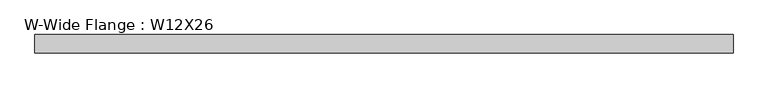
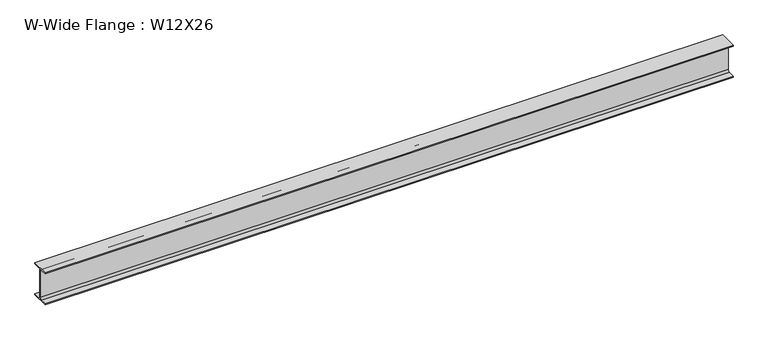
"""IFC4 building model written with IfcOpenShell, lengths in millimetres: beam geometry, W-Wide Flange : W12X26."""

from ifc_helpers import new_model, si_unit, point, frame, frame_2d, origin, place, context, project, spatial, polyline, circle_curve, trimmed, segment, composite_curve, outline, extrude, source, transform, mapped, element, save


def w_wide_flange_w12x26_2b793ae1(model_context):
    return source(origin(), model_context, "Body", "SweptSolid", [
        extrude(outline(composite_curve([segment(polyline([(82.4011719, -145.5539063), (82.4011719, -155.178125), (-82.4011719, -155.178125), (-82.4011719, -145.5539063), (-20.2902344, -145.5539063)]), True, "CONTINUOUS"), segment(trimmed(circle_curve(frame_2d((-20.2902344, -128.190625)), 17.3632812), [point((-20.2902344, -145.5539063))], [point((-2.9269531, -128.190625))], True, "CARTESIAN"), True, "CONTINUOUS"), segment(polyline([(-2.9269531, -128.190625), (-2.9269531, 128.190625)]), True, "CONTINUOUS"), segment(trimmed(circle_curve(frame_2d((-20.2902344, 128.190625)), 17.3632812), [point((-2.9269531, 128.190625))], [point((-20.2902344, 145.5539062))], True, "CARTESIAN"), True, "CONTINUOUS"), segment(polyline([(-20.2902344, 145.5539062), (-82.4011719, 145.5539062), (-82.4011719, 155.178125), (82.4011719, 155.178125), (82.4011719, 145.5539062), (20.2902344, 145.5539062)]), True, "CONTINUOUS"), segment(trimmed(circle_curve(frame_2d((20.2902344, 128.190625)), 17.3632812), [point((20.2902344, 145.5539062))], [point((2.9269531, 128.190625))], True, "CARTESIAN"), True, "CONTINUOUS"), segment(polyline([(2.9269531, 128.190625), (2.9269531, -128.190625)]), True, "CONTINUOUS"), segment(trimmed(circle_curve(frame_2d((20.2902344, -128.190625)), 17.3632812), [point((2.9269531, -128.190625))], [point((20.2902344, -145.5539063))], True, "CARTESIAN"), True, "CONTINUOUS"), segment(polyline([(20.2902344, -145.5539063), (82.4011719, -145.5539063)]), True, "CONTINUOUS")], self_intersect=False)), frame((-3159.4630915, 0.0, 0.0), z_axis=(1.0, 0.0, 0.0), x_axis=(0.0, 1.0, 0.0)), (0.0, 0.0, 1.0), 6318.926183),
    ])


if __name__ == "__main__":
    model = new_model("IFC4")
    model_context = context("Model", 3, world=origin())
    ifc_project = project(units=[si_unit("LENGTHUNIT", "METRE", prefix="MILLI")], contexts=[model_context])
    site = spatial("IfcSite", under=ifc_project)
    building = spatial("IfcBuilding", under=site)
    placement = place(None, origin())
    w_wide_flange_w12x26_shape = w_wide_flange_w12x26_2b793ae1(model_context)
    element("IfcBeam", 1, ObjectType="W-Wide Flange : W12X26", at=placement, inside=building, context=model_context, shape_type="MappedRepresentation", body=[
        mapped(w_wide_flange_w12x26_shape, transform((0.0, 0.0, 0.0), x_axis=(1.0, 0.0, 0.0), y_axis=(0.0, 1.0, 0.0), z_axis=(0.0, 0.0, 1.0))),
    ])
    save(model, "model.ifc")

# Revit data of these elements
# Type "W-Wide Flange : W12X26"
#   Assembly Code = "B10"
#   W = 26
#   Length [instance default] = 5' - 0"
#   bf = 0' - 6 125/256"
#   d = 1' - 0 7/32"
#   k = 0' - 1 1/16"
#   k2 = 0' - 0 175/256"
#   tf = 0' - 0 97/256"
#   tw = 0' - 0 59/256"
#   A = 0.053125 SF
#   Structural Material [instance default] = none
# Element 1 (IfcBeam, "W-Wide Flange : W12X26")
#   Structural Material = Dark metal
#   Materials on its faces: "Dark metal"
# Materials
#   "Dark metal": class "Generic", colour RGB 44 29 29, transparency 0, Cost = 0
